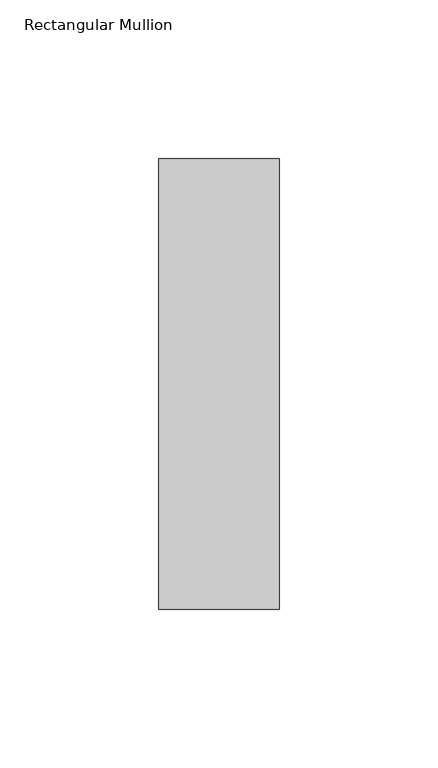
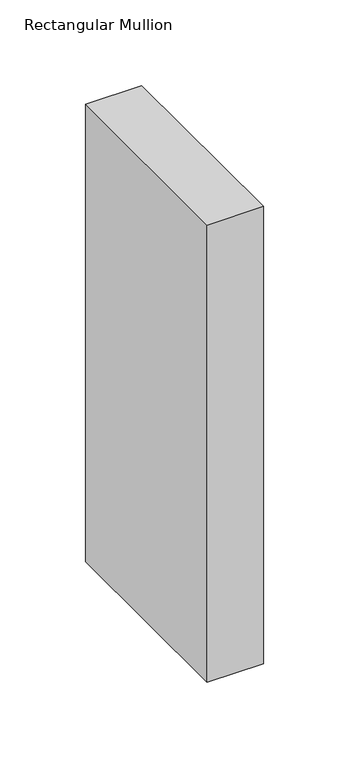
"""IFC4 building model written with IfcOpenShell, lengths in millimetres: member geometry, Rectangular Mullion : NLRS_21_CWM_hsb-regel 38x142_gen_rsf."""

from ifc_helpers import new_model, si_unit, frame, origin, place, context, project, spatial, polyline, outline, extrude, source, transform, mapped, element, save


def rectangular_mullion_66002bf8(model_context):
    return source(origin(), model_context, "Body", "SweptSolid", [
        extrude(outline(polyline([(-38.0, -71.0), (-38.0, 71.0), (0.0, 71.0), (0.0, -71.0), (-38.0, -71.0)])), frame((0.0, 0.0, -326.0000003), z_axis=(0.0, 0.0, 1.0), x_axis=(1.0, 0.0, 0.0)), (0.0, 0.0, 1.0), 326.0000003),
    ])


if __name__ == "__main__":
    model = new_model("IFC4")
    model_context = context("Model", 3, world=origin())
    ifc_project = project(units=[si_unit("LENGTHUNIT", "METRE", prefix="MILLI")], contexts=[model_context])
    site = spatial("IfcSite", under=ifc_project)
    building = spatial("IfcBuilding", under=site)
    placement = place(None, origin())
    rectangular_mullion_shape = rectangular_mullion_66002bf8(model_context)
    element("IfcMember", 1, ObjectType="Rectangular Mullion : NLRS_21_CWM_hsb-regel 38x142_gen_rsf", at=placement, inside=building, context=model_context, shape_type="MappedRepresentation", body=[
        mapped(rectangular_mullion_shape, transform((0.0, 0.0, 0.0), x_axis=(1.0, 0.0, 0.0), y_axis=(0.0, 1.0, 0.0), z_axis=(0.0, 0.0, 1.0))),
    ])
    save(model, "model.ifc")

# Revit data of these elements
# Type "Rectangular Mullion : NLRS_21_CWM_hsb-regel 38x142_gen_rsf"
#   Export Type to IFC As = "IfcWall"
#   Type IfcGUID = "07M7mRoiH1CR8m_RSKIwpF"
#   Assembly Code = "21.10"
#   built-in parameter 1007322 = 0.465879 (stored number, unit not read)
#   built-in parameter 1007321 = 0.062336 (stored number, unit not read)
#   built-in parameter 1007320 = 0.062336 (stored number, unit not read)
# Element 1 (IfcMember, "Rectangular Mullion : NLRS_21_CWM_hsb-regel 38x142_gen_rsf")
#   Materials on its faces: "NLRS_i2_hout naaldhout vuren_gen_rsf"
# Materials
#   "NLRS_i2_hout naaldhout vuren_gen_rsf": class "I - Hout", colour RGB 234 199 147, transparency 0, Keynote = "i2", Manufacturer = "Revit Standards Foundation", URL = "www.revitstandards.org", Description = "hout vuren", Cost = 0
